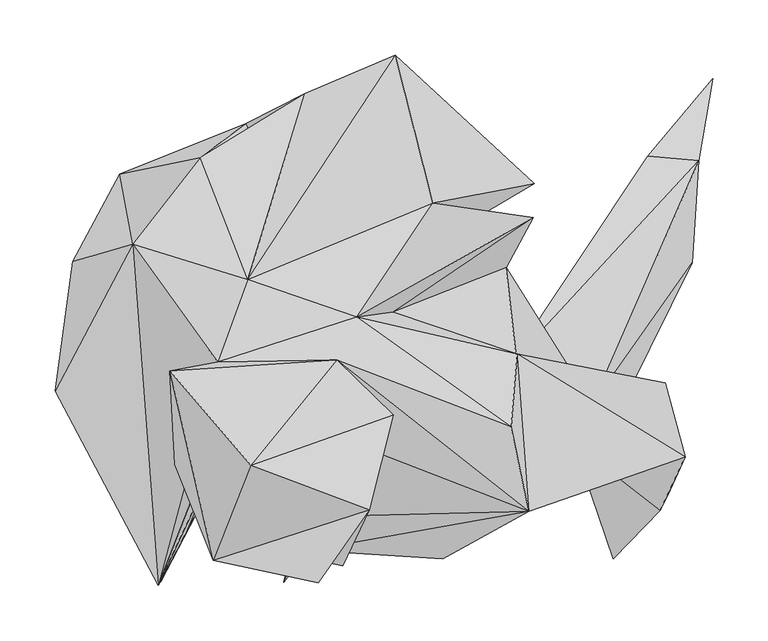
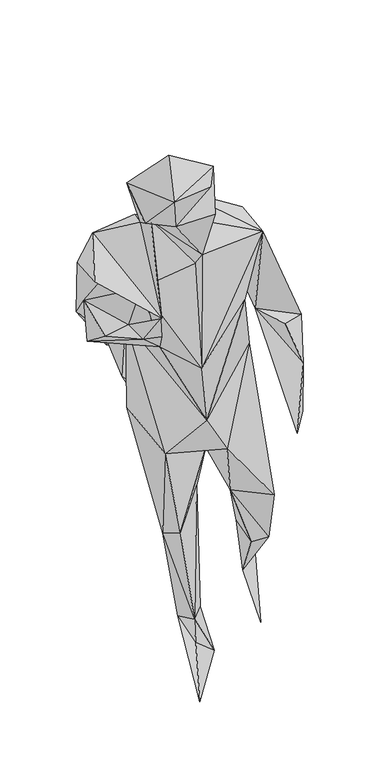
"""IFC4 building model written with IfcOpenShell, lengths in millimetres: geographic element geometry, Enscape AssetDefinition - Andres 001 Walking : Enscape AssetDefinition - Andres 001 Walking."""

from ifc_helpers import new_model, si_unit, origin, place, context, project, spatial, faceted_brep, source, transform, mapped, element, save


def geographic_element_ac00a26d(model_context):
    return source(origin(), model_context, "Body", "Brep", [
        faceted_brep([(-71.8359053, 109.1381237, 1179.3904305), (-105.8252826, 243.6383814, 810.2130294), (-239.8703098, 40.0509574, 1370.9090948), (-187.9559755, 208.9042962, 1076.5315294), (-241.4339483, 181.6816181, 880.3887367), (-224.4961709, 89.4911811, 924.4329333), (20.2184599, 127.2684336, 776.3175964), (-90.307638, 182.7999204, 744.9631691), (-156.7672938, 173.3191162, 738.5379076), (-282.880336, 150.814563, 1224.3821621), (-221.7449397, 137.8551573, 963.8728499), (-355.9557498, 135.7150674, 1050.8378744), (-344.2507088, 72.2466037, 1330.6974173), (-298.4276414, 99.8082384, 995.316267), (-381.2090158, 53.5150915, 1145.6731558), (-380.0016642, -30.9709627, 1256.5332651), (-398.418963, 56.0263135, 1267.171979), (-307.5917661, -111.8522212, 1257.8568459), (-414.5427644, -61.2838082, 1283.4738493), (-321.026206, -237.893492, 1245.100379), (-266.8950558, -34.7464569, 1400.3955126), (-269.8565722, -128.1096339, 1283.0557823), (-258.0303252, -75.9825185, 1426.6064167), (-297.0817089, -192.5108284, 1216.2473202), (-179.9076796, -164.5780653, 1321.790576), (-305.4170012, -42.5052792, 1101.5473604), (-184.5021099, -206.0046345, 1023.016572), (-266.4868236, -134.7204596, 1074.7749805), (-165.7656431, -174.9223322, 1349.7776985), (-62.9835278, -213.639766, 1196.5385675), (-165.3302014, -198.0528384, 849.6454358), (15.2504398, -170.3848243, 1355.39639), (-256.8996549, -198.1146783, 1482.6401472), (-153.6127925, -220.1318294, 1497.4848032), (-117.513001, -119.1657111, 1400.3288746), (-159.2463553, -33.2817845, 1463.5621309), (-129.7128499, -169.3283617, 1607.4392796), (-237.2551858, -128.7850589, 1655.5806398), (-310.4889393, -43.3563739, 1543.320179), (-107.5720042, -82.8729272, 1541.1999226), (-0.8931552, -93.7045962, 1390.5931711), (-271.0268497, -214.8495913, 1573.6107826), (-306.0256541, -127.9438585, 1468.2160616), (-175.9194136, -235.5455607, 1601.0288), (-140.7746226, 5.6582987, 1347.9220867), (4.6018525, -27.5170971, 1290.1268005), (-108.259812, 10.3096338, 1050.7018566), (19.1051085, 96.3494256, 936.2517595), (12.5536546, -105.7461053, 971.562326), (-5.3193453, 50.860364, 836.3495469), (-74.1863102, 71.3534504, 904.7612548), (-121.6571406, 82.6601535, 824.9092102), (72.9344115, -73.3277947, 538.2138491), (-101.8642262, 48.8563292, 721.3279605), (-184.9202365, 55.6848869, 785.2244377), (-192.4662888, 65.6753629, 726.6522646), (-273.5702097, 42.9308265, 876.3782978), (-261.0042095, 48.3986214, 1038.8656855), (-355.1689684, 80.7674527, 992.2360182), (-291.5248573, -10.7821887, 820.4360604), (-253.5299063, -138.6221349, 740.4677272), (-201.2320757, -37.1537693, 414.6095812), (-88.741526, -60.2595247, 655.7787657), (-185.5560839, -99.5558798, 447.9507208), (-105.8995128, -198.7455934, 740.4206991), (67.2167316, -138.958618, 501.7157197), (-5.831487, -41.4216183, 483.3924174), (8.2561187, -74.611865, 1153.4221172), (45.7859561, -79.3695822, 1051.7311096), (138.7953311, -54.0272333, 1037.5716686), (157.0023298, -121.0880876, 1018.5779333), (134.3889236, -169.4372296, 904.6103358), (97.5419506, -141.1407888, 1022.3163366), (143.5134709, -151.1362046, 741.3806319), (91.6980952, -213.4665698, 729.1758657), (163.5686308, 55.679936, 219.2757726), (169.4768071, 148.1895447, 204.3939978), (107.5843796, 91.0622403, 115.5757681), (104.4521481, 43.3266871, 232.09171), (123.2850999, 152.0343125, 226.5521586), (119.6159944, 20.0230051, -9.1171106), (182.206139, 222.3906964, 141.4475888), (-93.6229527, -22.0839418, 516.6816115), (-127.9760152, -71.133256, 143.0112273), (-69.9852705, 0.8659399, 118.1191579), (-48.1437854, -32.5519219, -4.3272255), (-159.3750119, -41.5329523, 145.982638), (-135.1286918, -89.3476829, 84.5701694), (-207.2491199, -234.6647829, 13.3775352), (-297.0817089, -192.5108284, 1207.8748941), (-318.4852898, -234.6524, 1184.6231222), (-326.8972635, -156.1141163, 1131.8849325), (-362.9970551, -23.9716917, 1074.0722418)], [[[0, 1, 2]], [[1, 3, 2]], [[3, 1, 4]], [[1, 5, 4]], [[1, 0, 6]], [[6, 7, 1]], [[1, 7, 8]], [[8, 5, 1]], [[9, 3, 10]], [[9, 2, 3]], [[4, 10, 3]], [[9, 10, 4]], [[9, 11, 12]], [[4, 11, 9]], [[9, 12, 2]], [[11, 13, 14]], [[11, 4, 13]], [[14, 15, 11]], [[11, 16, 12]], [[15, 16, 11]], [[17, 15, 14]], [[17, 18, 15]], [[18, 16, 15]], [[16, 18, 12]], [[19, 12, 18]], [[17, 19, 18]], [[19, 20, 12]], [[12, 20, 2]], [[21, 22, 19]], [[22, 20, 19]], [[23, 21, 19]], [[19, 17, 23]], [[21, 17, 22]], [[17, 21, 23]], [[22, 17, 24]], [[25, 17, 14]], [[24, 17, 26]], [[27, 17, 25]], [[17, 27, 26]], [[24, 26, 28]], [[24, 28, 22]], [[29, 26, 30]], [[28, 26, 31]], [[26, 27, 30]], [[26, 29, 31]], [[28, 32, 22]], [[32, 28, 33]], [[33, 28, 34]], [[28, 31, 34]], [[35, 36, 33]], [[33, 36, 32]], [[33, 34, 35]], [[31, 35, 34]], [[37, 35, 38]], [[38, 35, 20]], [[37, 39, 35]], [[39, 36, 35]], [[40, 35, 31]], [[20, 35, 40]], [[38, 41, 37]], [[41, 38, 42]], [[20, 42, 38]], [[41, 36, 37]], [[36, 39, 37]], [[41, 42, 32]], [[41, 32, 43]], [[43, 36, 41]], [[43, 32, 36]], [[22, 32, 42]], [[22, 42, 20]], [[40, 44, 20]], [[20, 44, 2]], [[45, 40, 31]], [[45, 44, 40]], [[45, 46, 44]], [[44, 46, 47]], [[0, 44, 47]], [[2, 44, 0]], [[46, 45, 48]], [[48, 49, 46]], [[47, 46, 49]], [[49, 50, 47]], [[47, 50, 0]], [[6, 0, 50]], [[51, 7, 50]], [[6, 50, 7]], [[49, 51, 50]], [[52, 53, 49]], [[52, 49, 48]], [[51, 49, 53]], [[51, 53, 54]], [[7, 51, 54]], [[7, 55, 8]], [[7, 54, 55]], [[8, 55, 5]], [[55, 54, 56]], [[5, 55, 56]], [[13, 4, 5]], [[13, 5, 56]], [[57, 56, 54]], [[57, 13, 56]], [[27, 58, 13]], [[14, 13, 58]], [[57, 27, 13]], [[59, 57, 54]], [[27, 57, 30]], [[30, 57, 60]], [[57, 59, 60]], [[54, 61, 59]], [[59, 61, 60]], [[62, 60, 63]], [[64, 60, 62]], [[64, 30, 60]], [[60, 61, 63]], [[29, 30, 48]], [[30, 64, 48]], [[48, 64, 65]], [[64, 62, 66]], [[66, 65, 64]], [[48, 67, 29]], [[65, 52, 48]], [[67, 48, 45]], [[31, 29, 67]], [[31, 67, 68]], [[69, 68, 67]], [[67, 45, 69]], [[31, 70, 45]], [[45, 70, 69]], [[31, 68, 70]], [[71, 70, 72]], [[73, 70, 71]], [[69, 70, 73]], [[68, 72, 70]], [[68, 69, 73]], [[73, 74, 68]], [[71, 68, 74]], [[68, 71, 72]], [[71, 74, 73]], [[66, 75, 65]], [[65, 75, 52]], [[75, 76, 52]], [[75, 77, 76]], [[78, 75, 66]], [[78, 77, 75]], [[52, 66, 62]], [[76, 66, 52]], [[52, 62, 53]], [[79, 78, 66]], [[76, 79, 66]], [[77, 80, 76]], [[76, 80, 81]], [[81, 79, 76]], [[78, 79, 77]], [[77, 79, 81]], [[77, 81, 80]], [[53, 82, 54]], [[62, 82, 53]], [[82, 62, 63]], [[63, 83, 82]], [[82, 84, 61]], [[82, 61, 54]], [[83, 84, 82]], [[63, 61, 83]], [[84, 83, 85]], [[83, 61, 86]], [[87, 83, 86]], [[87, 85, 83]], [[86, 61, 84]], [[86, 84, 85]], [[85, 87, 88]], [[85, 88, 86]], [[88, 87, 86]], [[27, 89, 90]], [[91, 58, 27]], [[91, 27, 90]], [[25, 89, 27]], [[90, 89, 91]], [[91, 89, 25]], [[91, 92, 58]], [[92, 91, 25]], [[92, 14, 58]], [[92, 25, 14]]]),
    ])


if __name__ == "__main__":
    model = new_model("IFC4")
    model_context = context("Model", 3, world=origin())
    ifc_project = project(units=[si_unit("LENGTHUNIT", "METRE", prefix="MILLI")], contexts=[model_context])
    site = spatial("IfcSite", under=ifc_project)
    building = spatial("IfcBuilding", under=site)
    placement = place(None, origin())
    geographic_element_shape = geographic_element_ac00a26d(model_context)
    element("IfcGeographicElement", 1, ObjectType="Enscape AssetDefinition - Andres 001 Walking : Enscape AssetDefinition - Andres 001 Walking", at=placement, inside=building, context=model_context, shape_type="MappedRepresentation", body=[
        mapped(geographic_element_shape, transform((0.0, 0.0, 0.0), x_axis=(1.0, 0.0, 0.0), y_axis=(0.0, 1.0, 0.0), z_axis=(0.0, 0.0, 1.0))),
    ])
    save(model, "model.ifc")

# Revit data of these elements
# Type "Enscape AssetDefinition - Andres 001 Walking : Enscape AssetDefinition - Andres 001 Walking"
#   EnscapeAssetSource = "REMOTE"
#   EnscapeAssetId = "efe3b603-d727-4329-9d41-8c8ad7c2fe4c"
#   Height = 1655.581 mm
#   EnscapeNativeAssetHeight = 1655.581 mm
#   Default Elevation = 0
